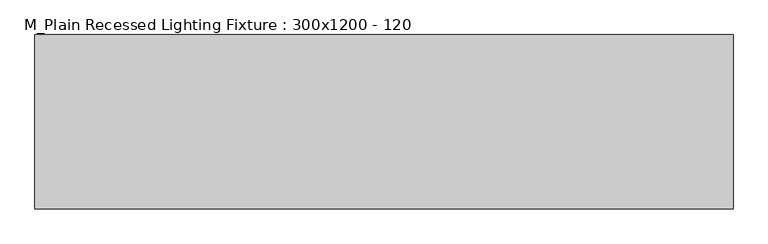
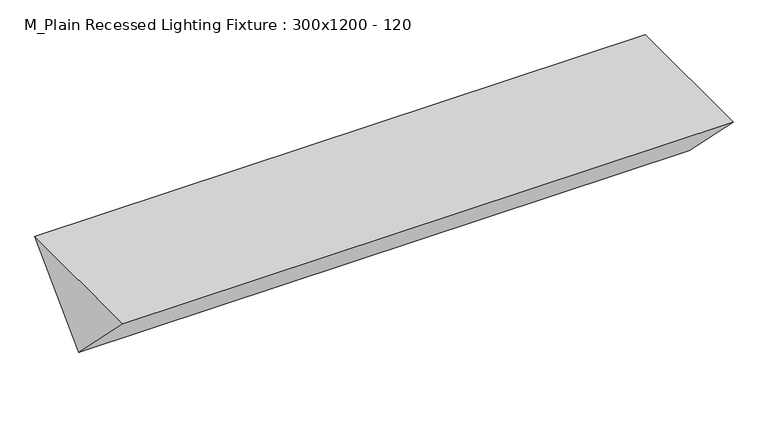
"""IFC4 building model written with IfcOpenShell, lengths in millimetres: light fixture geometry, M_Plain Recessed Lighting Fixture : 300x1200 - 120."""

from ifc_helpers import new_model, si_unit, frame, origin, place, context, project, spatial, polyline, outline, extrude, source, transform, mapped, element, save


def m_plain_recessed_lighting_fixture_300x1200_120_e46e8774(model_context):
    return source(origin(), model_context, "Body", "SweptSolid", [
        extrude(outline(polyline([(-300.0, 0.0), (0.0, 0.0), (-150.0, -150.0), (-300.0, 0.0)])), frame((0.0, 0.0, 0.0), z_axis=(1.0, 0.0, 0.0), x_axis=(0.0, 1.0, 0.0)), (0.0, 0.0, 1.0), 1200.0),
    ])


if __name__ == "__main__":
    model = new_model("IFC4")
    model_context = context("Model", 3, world=origin())
    ifc_project = project(units=[si_unit("LENGTHUNIT", "METRE", prefix="MILLI")], contexts=[model_context])
    site = spatial("IfcSite", under=ifc_project)
    building = spatial("IfcBuilding", under=site)
    placement = place(None, origin())
    m_plain_recessed_lighting_fixture_300x1200_120_shape = m_plain_recessed_lighting_fixture_300x1200_120_e46e8774(model_context)
    element("IfcLightFixture", 1, ObjectType="M_Plain Recessed Lighting Fixture : 300x1200 - 120", at=placement, inside=building, context=model_context, shape_type="MappedRepresentation", body=[
        mapped(m_plain_recessed_lighting_fixture_300x1200_120_shape, transform((0.0, 0.0, 0.0), x_axis=(1.0, 0.0, 0.0), y_axis=(0.0, 1.0, 0.0), z_axis=(0.0, 0.0, 1.0))),
    ])
    save(model, "model.ifc")

# Revit data of these elements
# Type "M_Plain Recessed Lighting Fixture : 300x1200 - 120"
#   Photometric Web File = "1x42A12.ies"
#   Width = 300 mm
#   Wattage = 64 W
#   built-in parameter 1150110 = 1 (stored number, unit not read)
#   built-in parameter 1150109 = 1 (stored number, unit not read)
#   built-in parameter 1150113 = 1 (stored number, unit not read)
#   Tilt Angle = -90.00°
#   Lumens = 5699.84 lm
#   built-in parameter 1114217 = 0.88 (stored number, unit not read)
#   built-in parameter 1150115 = 1 (stored number, unit not read)
#   built-in parameter 1150105 = 453.579 (stored number, unit not read)
#   Length = 1200 mm
#   built-in parameter 1150112 = 1 (stored number, unit not read)
#   built-in parameter 1150114 = 1 (stored number, unit not read)
#   built-in parameter 1150107 = 4230 (stored number, unit not read)
#   built-in parameter 1150106 = 4.53579 (stored number, unit not read)
#   Emit from Rectangle Width = 300 mm
#   Emit from Rectangle Length = 1200 mm
#   built-in parameter 1150104 = 8.27394 (stored number, unit not read)
#   Depth = 150 mm
#   Default Elevation = 2000 mm
#   Ballast Voltage = 120 V
#   built-in parameter 1114218 = 0.88 (stored number, unit not read)
#   built-in parameter 1150133 = 10 (stored number, unit not read)
#   Apparent Load = 64 VA
#   built-in parameter 1150134 = 8
#   built-in parameter 1150137 = 1
#   Color Filter = 16777215
#   built-in parameter 1140040 [instance default] = 1
#   Load Classification = Lighting - Dwelling Unit
#   Emit Shape Visible in Rendering = no
#   Dimming Lamp Color Temperature Shift = (empty or 0)
#   Assembly Code = ""
